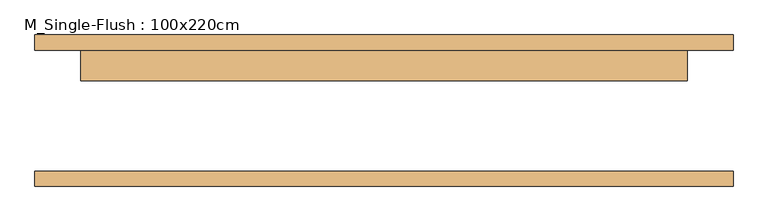
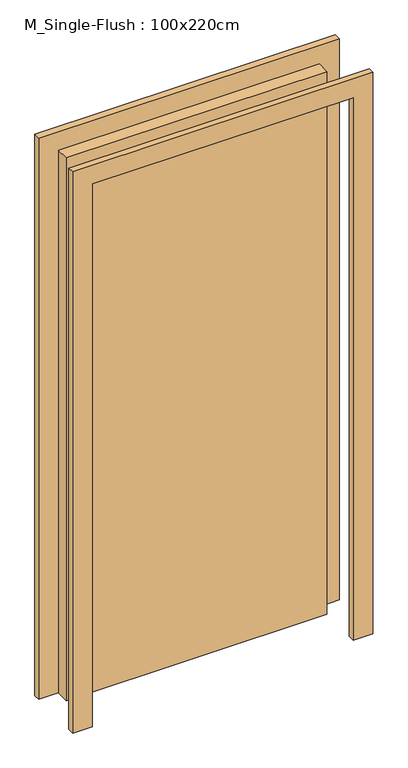
"""IFC4 building model written with IfcOpenShell, lengths in millimetres: door geometry, M_Single-Flush : 100x220cm."""

from ifc_helpers import new_model, si_unit, frame, origin, origin_with_axes, place, context, project, spatial, polyline, outline, extrude, source, transform, mapped, element, save


def m_single_flush_100x220cm_5dd7b505(model_context):
    return source(origin(), model_context, "Body", "SweptSolid", [
        extrude(outline(polyline([(2276.0, -576.0), (0.0, -576.0), (0.0, -500.0), (2200.0, -500.0), (2200.0, 500.0), (0.0, 500.0), (0.0, 576.0), (2276.0, 576.0), (2276.0, -576.0)])), frame((0.0, 100.0, 0.0), z_axis=(0.0, 1.0, 0.0), x_axis=(0.0, 0.0, 1.0)), (0.0, 0.0, 1.0), 25.0),
        extrude(outline(polyline([(2276.0, 576.0), (2276.0, -576.0), (0.0, -576.0), (0.0, -500.0), (2200.0, -500.0), (2200.0, 500.0), (0.0, 500.0), (0.0, 576.0), (2276.0, 576.0)])), frame((0.0, -125.0, 0.0), z_axis=(0.0, 1.0, 0.0), x_axis=(0.0, 0.0, 1.0)), (0.0, 0.0, 1.0), 25.0),
        extrude(outline(polyline([(500.0, 49.0), (-500.0, 49.0), (-500.0, 100.0), (500.0, 100.0), (500.0, 49.0)])), origin_with_axes(), (0.0, 0.0, 1.0), 2200.0),
    ])


if __name__ == "__main__":
    model = new_model("IFC4")
    model_context = context("Model", 3, world=origin())
    ifc_project = project(units=[si_unit("LENGTHUNIT", "METRE", prefix="MILLI")], contexts=[model_context])
    site = spatial("IfcSite", under=ifc_project)
    building = spatial("IfcBuilding", under=site)
    placement = place(None, origin())
    m_single_flush_100x220cm_shape = m_single_flush_100x220cm_5dd7b505(model_context)
    element("IfcDoor", 1, ObjectType="M_Single-Flush : 100x220cm", at=placement, inside=building, context=model_context, shape_type="MappedRepresentation", body=[
        mapped(m_single_flush_100x220cm_shape, transform((0.0, 0.0, 0.0), x_axis=(1.0, 0.0, 0.0), y_axis=(0.0, 1.0, 0.0), z_axis=(0.0, 0.0, 1.0))),
    ])
    save(model, "model.ifc")

# Revit data of these elements
# Type "M_Single-Flush : 100x220cm"
#   Type Mark = "44"
#   Construction Type Id = "MDOOR"
#   Analytic Construction = "Metal"
#   Thickness = 5.10 cm
#   Heat Transfer Coefficient (U) = 3.7021 W/(m²·K)
#   Height = 220.00 cm
#   Trim Projection Ext = 2.50 cm
#   Trim Projection Int = 2.50 cm
#   Trim Width = 7.60 cm
#   Width = 100.00 cm
#   Define Thermal Properties by = 1
#   Door Material = Door - Panel
#   Frame Material = Door - Frame
#   Visual Light Transmittance = 0
#   Solar Heat Gain Coefficient = 0
#   Function = (empty or 0)
#   Wall Closure = (empty or 0)
# Element 1 (IfcDoor, "M_Single-Flush : 100x220cm")
#   Materials on its faces: "Door - Frame", "Door - Panel"
# Materials
#   "Door - Panel": class "Wood", colour RGB 210 159 95, transparency 0, Cost = 0
#   "Door - Frame": class "Miscellaneous", colour RGB 118 70 51, transparency 0, Cost = 0
